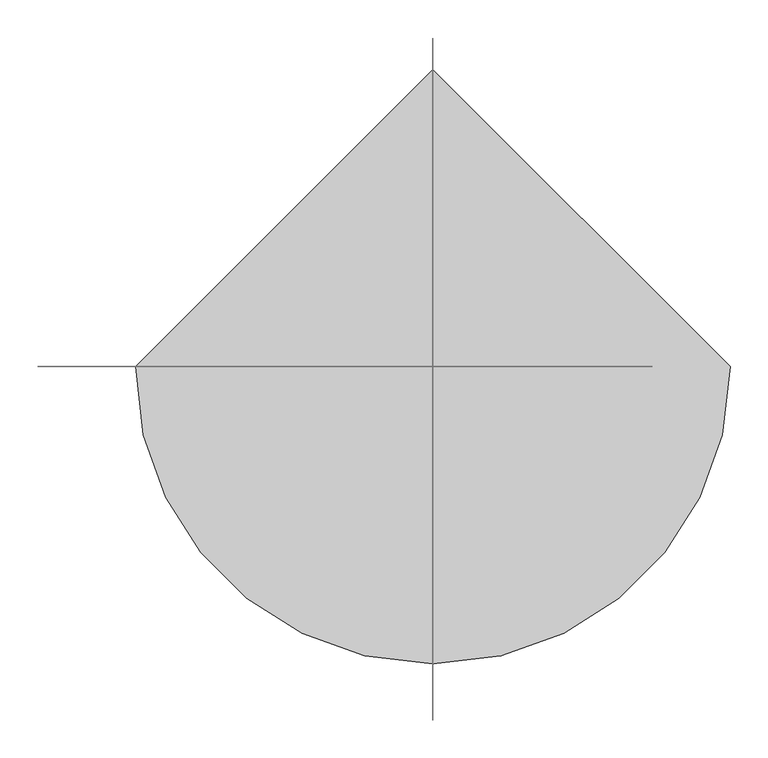
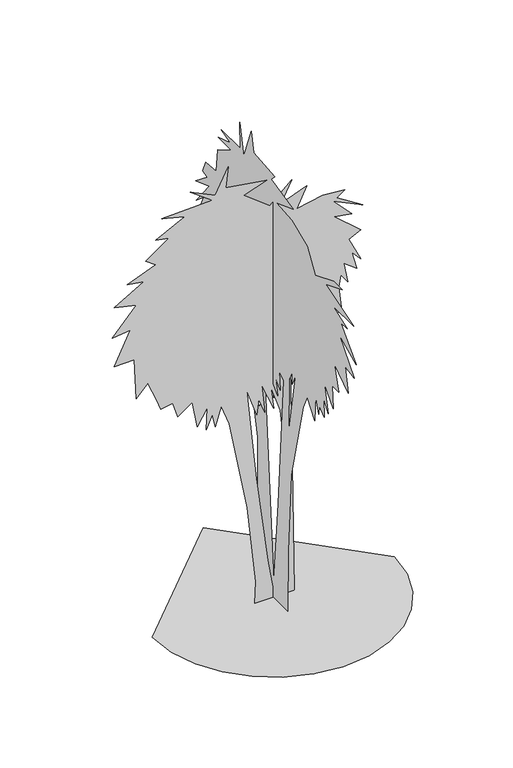
"""IFC4 building model written with IfcOpenShell, lengths in millimetres: proxy geometry, buddha belly bamboo 26099 : buddha belly bamboo 26099."""

from ifc_helpers import new_model, si_unit, origin, place, context, project, spatial, triangles, source, transform, mapped, element, save


def entourage_82ff1ee0(model_context):
    return source(origin(), model_context, "Body", "Tessellation", [
        triangles([(0.0, 68.9771396, 618.8468193), (0.0, 81.3218167, 600.9474395), (0.0, 100.5519475, 725.9461687), (0.0, -82.1358931, 0.0), (0.0, -83.3197871, 207.8534466), (0.0, -100.2098081, 479.1084738), (0.0, -168.6723352, 751.584938), (0.0, -191.1077027, 799.6621634), (0.0, -232.7734371, 745.1765356), (0.0, -239.1833838, 834.9174242), (0.0, -255.2095495, 780.4317965), (0.0, -258.4124971, 812.4815844), (0.0, -287.2593374, 790.0457445), (0.0, -284.0538463, 850.9423182), (0.0, -309.6951954, 815.6870573), (0.0, -287.2593374, 905.4280186), (0.0, -335.3340011, 847.7368452), (0.0, -332.1310716, 924.6583855), (0.0, -367.3863324, 924.6583855), (0.0, -342.0142256, 1006.888468), (0.0, -421.8719965, 953.5051712), (0.0, -402.5171459, 1031.9253119), (0.0, -453.9217844, 1024.0157656), (0.0, -371.2242886, 1123.7185461), (0.0, -466.7411691, 1078.5013933), (0.0, -379.5681833, 1169.6164713), (0.0, -416.1264896, 1170.1726873), (0.0, -333.4594789, 1199.982205), (0.0, -450.7162751, 1200.2920698), (0.0, -293.6703014, 1248.3692951), (0.0, -386.6166993, 1286.8300289), (0.0, -338.5395103, 1286.8300289), (0.0, -235.9784014, 1245.1638222), (0.0, -189.6746325, 1315.3974712), (0.0, -104.9042436, 1353.6627228), (0.0, -18.0349252, 1360.5461689), (0.0, -110.9814616, 1395.8014297), (0.0, 10.8103129, 1424.6455994), (0.0, -8.4197106, 1443.8761116), (0.0, 108.6159538, 1455.4355804), (0.0, 122.9870424, 1520.7975792), (0.0, 164.6530312, 1408.6207054), (0.0, 187.0881443, 1511.1836311), (0.0, 183.8834162, 1424.6455994), (0.0, 292.8549624, 1421.4427425), (0.0, 240.050046, 1409.5376553), (0.0, 308.8798745, 1386.1848656), (0.0, 235.1638254, 1386.1848656), (0.0, 312.0853475, 1341.3156567), (0.0, 318.4963297, 1264.3941891), (0.0, 379.3903962, 1257.9832432), (0.0, 395.4152902, 1219.5225094), (0.0, 369.7764845, 1213.1140343), (0.0, 433.8786037, 1161.831336), (0.0, 358.9662068, 1188.3946856), (0.0, 430.6730945, 1097.7317602), (0.0, 389.0068514, 1132.9870211), (0.0, 421.0566393, 1065.6819723), (0.0, 353.7515905, 1126.5760752), (0.0, 417.8511663, 1014.3992741), (0.0, 385.8013784, 1049.6545349), (0.0, 315.2908204, 1120.1676727), (0.0, 382.5958692, 966.3245922), (0.0, 344.1351354, 1011.1963446), (0.0, 353.7515905, 943.8887524), (0.0, 328.1102414, 998.3743801), (0.0, 328.1102414, 918.2473669), (0.0, 315.2908204, 918.2473669), (0.0, 331.3157144, 873.3782307), (0.0, 283.2385072, 889.4031246), (0.0, 324.9047321, 799.6621634), (0.0, 289.6494713, 796.4566904), (0.0, 302.4714176, 713.1242043), (0.0, 280.0355596, 757.9959566), (0.0, 283.2385072, 687.4853622), (0.0, 254.3942104, 745.1765356), (0.0, 244.7792813, 655.435647), (0.0, 231.9590973, 709.9212748), (0.0, 219.1386771, 645.8191555), (0.0, 193.4985997, 671.4604683), (0.0, 174.2682328, 639.4082096), (0.0, 161.4480487, 757.9959566), (0.0, 135.8077261, 645.8191555), (0.0, 132.6024893, 697.0993103), (0.0, 87.4312912, 494.6812151), (0.0, 84.5267992, 0.0), (0.0, 42.8608059, 709.9212748), (0.0, -2.0096292, 684.2798893), (0.0, 20.4257563, 748.3820086), (0.0, -24.4450082, 703.5102562), (0.0, -14.8297941, 757.9959566), (0.0, -40.4701542, 732.3545712), (0.0, -34.0601984, 793.2512175), (0.0, -59.7005347, 777.2263235), (0.0, -26.9908557, 335.1155551), (0.0, -2.0096292, 56.0896632), (0.0, 46.0662925, 693.8938374), (0.0, -107.7764792, 834.9174242), (0.0, -107.7764792, 793.2512175), (0.0, -127.0066009, 838.1229698), (0.0, -87.4922522, 616.758938), (0.0, -88.5461032, 799.6621634), (1.2566193, -3.44e-05, 645.8191555), (-37.2039632, -4.13e-05, 738.7655897), (-27.588773, -3.44e-05, 642.6136826), (-46.8191535, -4.13e-05, 693.8938374), (-53.2293636, -3.44e-05, 642.6136826), (-85.2796511, -4.13e-05, 735.5600441), (-55.1696703, -2.75e-05, 424.8234515), (-17.6170944, -6.9e-06, 132.7480291), (1.1592355, 0.0, 15.9178056), (11.5905001, 0.0, 28.4353578), (19.935561, -6.9e-06, 174.4731985), (38.7117087, -2.75e-05, 468.6360025), (22.0217686, -3.44e-05, 631.3640059), (-8.3588267, -4.13e-05, 722.7406958), (-59.6393193, 0.0, 0.0), (-57.2560346, 0.0, 72.2466348), (-84.3771898, -2.06e-05, 335.1155551), (-142.9707881, -3.44e-05, 642.6136826), (-168.6113833, -4.13e-05, 713.1242043), (-187.8412415, -3.44e-05, 649.0246284), (-197.4566975, -4.13e-05, 693.8938374), (-216.6870644, -3.44e-05, 649.0246284), (-213.4818458, -4.13e-05, 722.7406958), (-245.5323785, -4.13e-05, 668.2549953), (-261.5570181, -4.13e-05, 757.9959566), (-309.6342253, -4.13e-05, 725.9461687), (-325.6591192, -4.81e-05, 777.2263235), (-364.1198894, -4.81e-05, 770.8153776), (-376.9393104, -4.81e-05, 806.0706385), (-405.7861324, -4.81e-05, 873.3782307), (-444.2443591, -4.81e-05, 834.9174242), (-450.655305, -5.5e-05, 969.5300652), (-514.7574243, -5.5e-05, 969.5300652), (-463.474726, -6.19e-05, 1075.2959204), (-521.165863, -6.19e-05, 1068.8849018), (-444.2443591, -6.88e-05, 1155.4229336), (-514.7574243, -6.88e-05, 1171.4478275), (-418.6055534, -6.88e-05, 1225.9334553), (-473.0911812, -7.57e-05, 1235.5474033), (-380.1447833, -7.57e-05, 1270.805135), (-412.1945712, -7.57e-05, 1293.238504), (-338.9001715, -8.25e-05, 1346.9494698), (-380.1447833, -8.25e-05, 1354.1350777), (-287.1983673, -8.25e-05, 1402.2123756), (-360.9144164, -8.25e-05, 1421.4401264), (-197.4566975, -8.25e-05, 1427.8512177), (-267.9680004, -8.94e-05, 1479.1313725), (-187.8412415, -8.25e-05, 1440.6731094), (-146.1757705, -8.94e-05, 1524.0030521), (-153.2237688, -8.25e-05, 1455.4355804), (-21.178765, -8.25e-05, 1434.2621635), (-94.8948436, -8.25e-05, 1408.6207054), (-11.5635259, -8.25e-05, 1344.5212749), (59.5745477, -8.25e-05, 1407.4498466), (23.691668, -7.57e-05, 1338.1101837), (108.2181855, -8.25e-05, 1370.1295956), (76.2893023, -7.57e-05, 1302.3062645), (160.5267932, -7.57e-05, 1319.5021626), (232.0200674, -7.57e-05, 1312.4688709), (205.3192808, -7.57e-05, 1295.4712166), (289.7104414, -7.57e-05, 1241.9583492), (193.5598241, -7.57e-05, 1286.8300289), (253.5961305, -6.88e-05, 1223.860762), (196.7647884, -7.57e-05, 1232.3444012), (283.3020026, -6.88e-05, 1158.6284065), (244.8404876, -6.88e-05, 1139.3980396), (283.3020026, -6.19e-05, 1059.2710264), (254.4551624, -6.19e-05, 1091.3208143), (270.4800563, -6.19e-05, 1030.424168), (228.8153393, -6.19e-05, 1062.4764994), (241.6355052, -5.5e-05, 995.1689072), (219.2001559, -6.19e-05, 1027.2212385), (212.7899367, -5.5e-05, 985.5549591), (222.4051383, -5.5e-05, 902.222473), (183.9443682, -5.5e-05, 895.8140705), (206.37999, -4.81e-05, 844.5313723), (155.099054, -4.81e-05, 857.3533367), (148.6891073, -4.81e-05, 783.6372694), (119.8432845, -4.81e-05, 796.4566904), (103.8178818, -4.81e-05, 770.8153776), (74.972822, -4.81e-05, 809.2761114), (71.7675898, -4.13e-05, 745.1765356), (55.7421917, -4.81e-05, 767.609832), (61.6606531, -2.75e-05, 431.0820448), (68.5626119, 0.0, 0.0), (-392.2986926, 0.0, 0.0), (-381.9278503, -89.8887448, 0.0), (-352.3901547, -172.4373852, 0.0), (-306.0528305, -245.2804135, 0.0), (-245.2804135, -306.0528305, 0.0), (-172.4373852, -352.3901547, 0.0), (-89.8887448, -381.9278503, 0.0), (1.71e-05, -392.2986926, 0.0), (89.8887448, -381.9278503, 0.0), (172.4373852, -352.3901547, 0.0), (245.2804135, -306.0528305, 0.0), (306.0528305, -245.2804135, 0.0), (352.3901547, -172.4373852, 0.0), (381.9278503, -89.8887448, 0.0), (392.2986926, 3.44e-05, 0.0), (-5.14e-05, 392.2986926, 0.0)], [[94, 4, 5], [4, 94, 95], [94, 5, 6], [42, 43, 44], [55, 56, 57], [59, 60, 61], [44, 45, 46], [4, 95, 96], [82, 83, 84], [62, 63, 64], [64, 65, 66], [28, 29, 30], [72, 73, 74], [46, 47, 48], [53, 54, 55], [76, 77, 78], [26, 27, 28], [24, 25, 26], [14, 15, 16], [10, 11, 12], [59, 61, 62], [57, 58, 59], [30, 31, 32], [30, 32, 33], [98, 99, 100], [74, 75, 76], [102, 98, 93], [40, 41, 42], [36, 37, 38], [86, 4, 96], [89, 90, 91], [80, 81, 82], [16, 17, 18], [102, 93, 94], [91, 92, 93], [87, 88, 89], [8, 9, 10], [22, 23, 24], [20, 21, 22], [12, 13, 14], [38, 39, 40], [101, 102, 94], [101, 94, 6], [101, 6, 7], [100, 101, 7], [100, 7, 8], [68, 69, 70], [78, 79, 80], [85, 86, 96], [85, 96, 97], [78, 80, 82], [70, 71, 72], [55, 57, 59], [18, 19, 20], [10, 12, 14], [51, 52, 53], [50, 51, 53], [76, 78, 82], [66, 67, 68], [44, 46, 48], [20, 22, 24], [42, 44, 48], [55, 59, 62], [50, 53, 55], [100, 8, 10], [10, 14, 16], [24, 26, 28], [62, 64, 66], [50, 55, 62], [16, 18, 20], [100, 10, 16], [38, 40, 42], [36, 38, 42], [48, 49, 50], [28, 30, 33], [72, 74, 76], [72, 76, 82], [70, 72, 82], [89, 91, 93], [3, 20, 24], [3, 24, 28], [3, 28, 33], [3, 33, 34], [3, 34, 35], [3, 35, 36], [3, 36, 42], [3, 42, 48], [3, 48, 50], [3, 50, 62], [3, 62, 66], [3, 66, 68], [3, 68, 70], [3, 70, 82], [3, 82, 84], [2, 3, 84], [2, 84, 85], [100, 16, 20], [1, 2, 85], [1, 85, 97], [3, 1, 97], [3, 97, 87], [3, 87, 89], [98, 100, 20], [98, 20, 3], [93, 98, 3], [93, 3, 89], [162, 163, 164], [148, 149, 150], [104, 105, 106], [116, 103, 104], [110, 117, 118], [168, 169, 170], [146, 147, 148], [150, 151, 152], [123, 124, 125], [155, 156, 157], [172, 173, 174], [106, 107, 108], [117, 110, 111], [187, 117, 111], [152, 153, 154], [121, 122, 123], [140, 141, 142], [144, 145, 146], [170, 171, 172], [164, 165, 166], [160, 161, 162], [183, 184, 185], [110, 118, 119], [109, 110, 119], [109, 119, 120], [108, 109, 120], [125, 126, 127], [136, 137, 138], [138, 139, 140], [157, 158, 159], [132, 133, 134], [108, 120, 121], [177, 178, 179], [104, 106, 108], [187, 111, 112], [134, 135, 136], [160, 162, 164], [166, 167, 168], [181, 182, 183], [186, 187, 112], [186, 112, 113], [186, 113, 114], [185, 186, 114], [185, 114, 115], [185, 115, 116], [179, 180, 181], [142, 143, 144], [127, 128, 129], [121, 123, 125], [175, 176, 177], [129, 130, 131], [179, 181, 183], [185, 116, 104], [150, 152, 154], [148, 150, 154], [159, 160, 164], [159, 164, 166], [168, 170, 172], [183, 185, 104], [166, 168, 172], [159, 166, 172], [159, 172, 174], [129, 131, 132], [159, 174, 175], [159, 175, 177], [159, 177, 179], [159, 179, 183], [159, 183, 104], [159, 104, 108], [157, 159, 108], [155, 157, 108], [155, 108, 121], [155, 121, 125], [155, 125, 127], [155, 127, 129], [155, 129, 132], [155, 132, 134], [155, 134, 136], [155, 136, 138], [155, 138, 140], [155, 140, 142], [154, 155, 142], [154, 142, 144], [148, 154, 144], [146, 148, 144], [202, 203, 188], [201, 202, 188], [201, 188, 189], [200, 201, 189], [200, 189, 190], [200, 190, 191], [199, 200, 191], [198, 199, 191], [198, 191, 192], [198, 192, 193], [198, 193, 194], [198, 194, 195], [198, 195, 196], [198, 196, 197]], closed=False),
    ])


if __name__ == "__main__":
    model = new_model("IFC4")
    model_context = context("Model", 3, world=origin())
    ifc_project = project(units=[si_unit("LENGTHUNIT", "METRE", prefix="MILLI")], contexts=[model_context])
    site = spatial("IfcSite", under=ifc_project)
    building = spatial("IfcBuilding", under=site)
    placement = place(None, origin())
    entourage_shape = entourage_82ff1ee0(model_context)
    element("IfcBuildingElementProxy", 1, Name="buddha belly bamboo 26099 : buddha belly bamboo 26099", ObjectType="buddha belly bamboo 26099 : buddha belly bamboo 26099", at=placement, inside=building, context=model_context, shape_type="MappedRepresentation", body=[
        mapped(entourage_shape, transform((0.0, 0.0, 0.0), x_axis=(1.0, 0.0, 0.0), y_axis=(0.0, 1.0, 0.0), z_axis=(0.0, 0.0, 1.0))),
    ])
    save(model, "model.ifc")

# Revit data of these elements
# Type "buddha belly bamboo 26099 : buddha belly bamboo 26099"
#   built-in parameter 1005195 = "RPC-16-FXGL-GN00-PMD1-0000-ST1L-LVER-AU"
#   Height = 0
